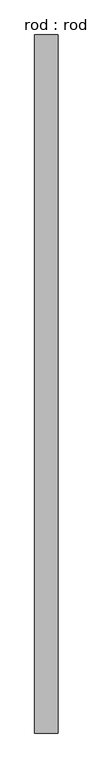
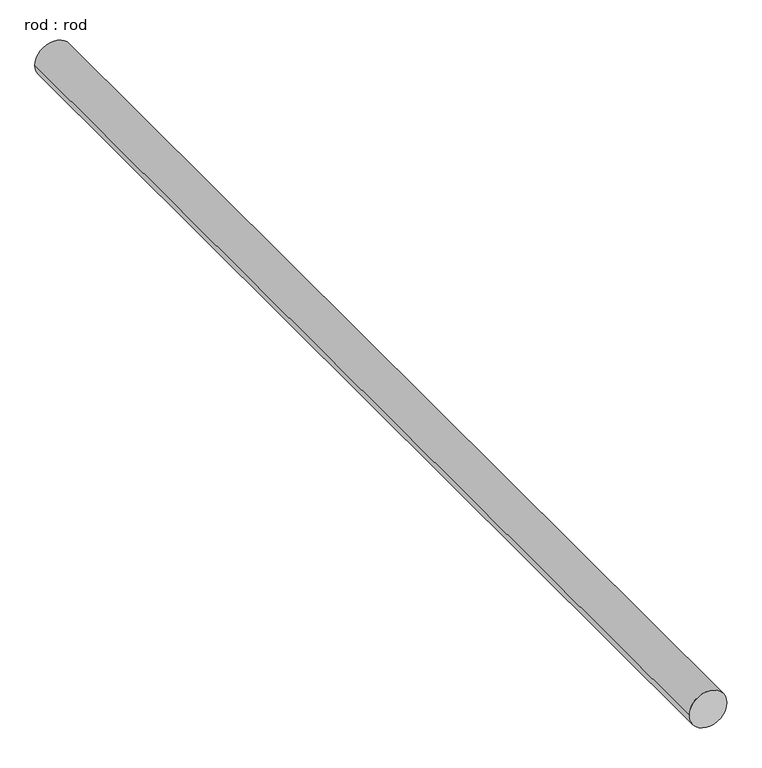
"""IFC4 building model written with IfcOpenShell, lengths in millimetres: proxy geometry, rod : rod."""

from ifc_helpers import new_model, si_unit, point, frame, frame_2d, origin, place, context, project, spatial, circle_curve, trimmed, segment, composite_curve, outline, extrude, source, transform, mapped, element, save


def rod_rod_8a8ab891(model_context):
    return source(origin(), model_context, "Body", "SweptSolid", [
        extrude(outline(composite_curve([segment(trimmed(circle_curve(frame_2d((0.0108462, 0.0)), 200.0), [point((0.0108462, 200.0))], [point((0.0108462, -200.0))], False, "CARTESIAN"), True, "CONTINUOUS"), segment(trimmed(circle_curve(frame_2d((0.0108462, 0.0)), 200.0), [point((0.0108462, -200.0))], [point((0.0108462, 200.0))], False, "CARTESIAN"), True, "CONTINUOUS")], self_intersect=False)), frame((0.0, -1907.2713847, 0.0), z_axis=(0.0, 1.0, 0.0), x_axis=(0.0, 0.0, 1.0)), (0.0, 0.0, 1.0), 12000.0),
    ])


if __name__ == "__main__":
    model = new_model("IFC4")
    model_context = context("Model", 3, world=origin())
    ifc_project = project(units=[si_unit("LENGTHUNIT", "METRE", prefix="MILLI")], contexts=[model_context])
    site = spatial("IfcSite", under=ifc_project)
    building = spatial("IfcBuilding", under=site)
    placement = place(None, origin())
    rod_rod_shape = rod_rod_8a8ab891(model_context)
    element("IfcBuildingElementProxy", 1, Name="rod : rod", ObjectType="rod : rod", at=placement, inside=building, context=model_context, shape_type="MappedRepresentation", body=[
        mapped(rod_rod_shape, transform((0.0, 0.0, 0.0), x_axis=(1.0, 0.0, 0.0), y_axis=(0.0, 1.0, 0.0), z_axis=(0.0, 0.0, 1.0))),
    ])
    save(model, "model.ifc")

# Revit data of these elements
# Type "rod : rod"
#   Default Elevation = 0
